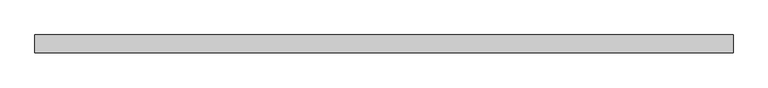
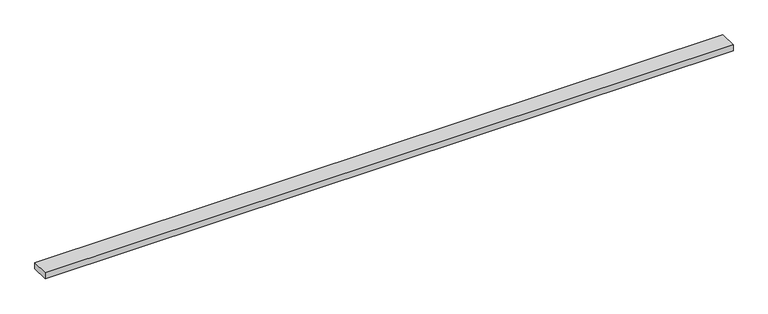
"""IFC4 building model written with IfcOpenShell, lengths in millimetres: proxy geometry, Generic Models 6:Generic Models 2:318829:Generic Models 2:318829 : Generic Models 6:Generic Models 2:318829:9 : Generic Models 6:Generic Models 2:318829:Generic Models 2:318829 : Generic Models 6:Generic Models 2:318829:300683."""

import ifcopenshell
import ifcopenshell.guid

model = None  # the IFC model being written
_history = None  # IfcOwnerHistory: only IFC2X3 demands one
_inside = {}  # id of a spatial element -> (the spatial element, [elements in it])
_under = {}  # id of a project, library or spatial element -> (it, [spatial elements below it])
_declared = {}  # id of a project -> (the project, [libraries it declares])
_typed = {}  # id of a type object -> (the type object, [elements of that type])
_made_of = {}  # id of a material, layer set ... -> (it, [elements and type objects made of it])


def new_model(schema):
    """Start an empty IFC model of exactly this schema.

    Asked for "IFC4X3", IfcOpenShell would pick the latest addendum, in which some entities
    have other attributes; the version numbers below select the first issue.
    IFC2X3 requires an IfcOwnerHistory on every rooted entity: one is made here for all.
    """
    global model, _history
    if schema == "IFC4X3":
        model = ifcopenshell.file(schema_version=(4, 3, 0, 0))
    else:
        model = ifcopenshell.file(schema=schema)
    _inside.clear()
    _under.clear()
    _declared.clear()
    _typed.clear()
    _made_of.clear()
    _history = None
    if model.schema == "IFC2X3":
        org = make("IfcOrganization", Name="unknown")
        user = make(
            "IfcPersonAndOrganization",
            ThePerson=make("IfcPerson", FamilyName="unknown"),
            TheOrganization=org,
        )
        app = make(
            "IfcApplication",
            ApplicationDeveloper=org,
            Version="unknown",
            ApplicationFullName="unknown",
            ApplicationIdentifier="unknown",
        )
        _history = make(
            "IfcOwnerHistory",
            OwningUser=user,
            OwningApplication=app,
            ChangeAction="ADDED",
            CreationDate=0,
        )
    return model


def make(cls, **values):
    """One entity of the class cls with the attributes given. An attribute that is None is left unset."""
    return model.create_entity(
        cls, **{name: value for name, value in values.items() if value is not None}
    )


def rooted(cls, **values):
    """An entity with a GlobalId (a new one), such as an element, a storey or a relation."""
    return make(cls, GlobalId=ifcopenshell.guid.new(), OwnerHistory=_history, **values)


def si_unit(unit_type, name, prefix=None):
    """IfcSIUnit, for example si_unit("LENGTHUNIT", "METRE", prefix="MILLI")."""
    return make("IfcSIUnit", UnitType=unit_type, Prefix=prefix, Name=name)


def assignment(units):
    """IfcUnitAssignment: the units of a project."""
    return None if units is None else make("IfcUnitAssignment", Units=units)


def point(xyz):
    """IfcCartesianPoint."""
    return None if xyz is None else make("IfcCartesianPoint", Coordinates=xyz)


def direction(xyz):
    """IfcDirection."""
    return None if xyz is None else make("IfcDirection", DirectionRatios=xyz)


def frame(location, z_axis=None, x_axis=None):
    """IfcAxis2Placement3D, a coordinate frame: its origin and axes. An axis left out is left unset."""
    return make(
        "IfcAxis2Placement3D",
        Location=point(location),
        Axis=direction(z_axis),
        RefDirection=direction(x_axis),
    )


def origin():
    """The frame at (0, 0, 0) with its axes left unset."""
    return frame((0.0, 0.0, 0.0))


def place(relative_to, where):
    """IfcLocalPlacement: puts the frame where relative to a parent placement (None: the world)."""
    return make(
        "IfcLocalPlacement", PlacementRelTo=relative_to, RelativePlacement=where
    )


def context(
    kind, dimensions, precision=None, world=None, true_north=None, identifier=None
):
    """IfcGeometricRepresentationContext, for example the 3D "Model" context."""
    return make(
        "IfcGeometricRepresentationContext",
        ContextIdentifier=identifier,
        ContextType=kind,
        CoordinateSpaceDimension=dimensions,
        Precision=precision,
        WorldCoordinateSystem=world,
        TrueNorth=true_north,
    )


def project(units=None, contexts=None):
    """IfcProject with its units and contexts."""
    return rooted(
        "IfcProject",
        Name="project",
        RepresentationContexts=contexts,
        UnitsInContext=assignment(units),
    )


def spatial(cls, under=None, at=None, **own):
    """A site, building, storey or space (cls), placed at a placement, below another one or the project."""
    s = rooted(cls, ObjectPlacement=at, **own)
    if under is not None:
        _under.setdefault(under.id(), (under, []))[1].append(s)
    return s


def polyline(points):
    """IfcPolyline through the points."""
    return make("IfcPolyline", Points=[point(p) for p in points])


def outline(outer, holes=None, kind="AREA"):
    """IfcArbitraryClosedProfileDef: a profile drawn as a closed curve; with holes, ...WithVoids."""
    if holes is None:
        return make("IfcArbitraryClosedProfileDef", ProfileType=kind, OuterCurve=outer)
    return make(
        "IfcArbitraryProfileDefWithVoids",
        ProfileType=kind,
        OuterCurve=outer,
        InnerCurves=holes,
    )


def extrude(swept, where, along, depth):
    """IfcExtrudedAreaSolid: the profile swept, set in the frame where, extruded along a direction by depth."""
    return make(
        "IfcExtrudedAreaSolid",
        SweptArea=swept,
        Position=where,
        ExtrudedDirection=direction(along),
        Depth=depth,
    )


def shape(context_of_items, identifier, shape_type, items):
    """IfcShapeRepresentation: the items that make up one representation, for example the "Body"."""
    return make(
        "IfcShapeRepresentation",
        ContextOfItems=context_of_items,
        RepresentationIdentifier=identifier,
        RepresentationType=shape_type,
        Items=items,
    )


def source(mapping_origin, context_of_items, identifier, shape_type, items):
    """IfcRepresentationMap: a shape defined once, which mapped items show again and again."""
    return make(
        "IfcRepresentationMap",
        MappingOrigin=mapping_origin,
        MappedRepresentation=shape(context_of_items, identifier, shape_type, items),
    )


def transform(
    local_origin,
    x_axis=None,
    y_axis=None,
    z_axis=None,
    scale=None,
    scale2=None,
    scale3=None,
    uniform=True,
):
    """IfcCartesianTransformationOperator3D, or its non-uniform kind. x_axis, y_axis, z_axis: its Axis1, 2, 3."""
    if uniform:
        return make(
            "IfcCartesianTransformationOperator3D",
            Axis1=direction(x_axis),
            Axis2=direction(y_axis),
            LocalOrigin=point(local_origin),
            Scale=scale,
            Axis3=direction(z_axis),
        )
    return make(
        "IfcCartesianTransformationOperator3DnonUniform",
        Axis1=direction(x_axis),
        Axis2=direction(y_axis),
        LocalOrigin=point(local_origin),
        Scale=scale,
        Axis3=direction(z_axis),
        Scale2=scale2,
        Scale3=scale3,
    )


def mapped(mapping_source, mapping_target):
    """IfcMappedItem: shows the shape of a source again, moved by a transform."""
    return make(
        "IfcMappedItem", MappingSource=mapping_source, MappingTarget=mapping_target
    )


def made_of(thing, what):
    """Note that an element or type object is made of a material, layer set ...; save() writes the relation."""
    if what is not None:
        _made_of.setdefault(what.id(), (what, []))[1].append(thing)
    return thing


def element(
    cls,
    number,
    at=None,
    inside=None,
    cuts=None,
    type_object=None,
    material=None,
    context=None,
    identifier="Body",
    shape_type=None,
    held_by="IfcProductDefinitionShape",
    body=None,
    shapes=None,
    **own,
):
    """One element of the class cls, such as IfcWall. Its Tag is "e" and its number.

    at: its placement. inside: the storey or other place that contains it. cuts: it is an
    opening in that element (IfcRelVoidsElement). A single representation is given by context,
    identifier, shape_type and body (its items); several are given by shapes. held_by: the class
    of the entity that holds the representations. save() writes the other relations.
    """
    e = rooted(cls, Tag="e%d" % number, ObjectPlacement=at, **own)
    if body is not None:
        shapes = [shape(context, identifier, shape_type, body)]
    if shapes is not None:
        e.Representation = make(held_by, Representations=shapes)
    if inside is not None:
        _inside.setdefault(inside.id(), (inside, []))[1].append(e)
    if cuts is not None:
        rooted(
            "IfcRelVoidsElement", RelatingBuildingElement=cuts, RelatedOpeningElement=e
        )
    if type_object is not None:
        _typed.setdefault(type_object.id(), (type_object, []))[1].append(e)
    return made_of(e, material)


def aggregate(whole, parts):
    """IfcRelAggregates: a whole, such as a stair, and the parts it consists of."""
    return rooted("IfcRelAggregates", RelatingObject=whole, RelatedObjects=parts)


def save(model, path):
    """Write the relations noted so far, then the file.

    IfcRelAggregates (storeys below a building ...), IfcRelContainedInSpatialStructure (elements
    in a storey), IfcRelDefinesByType, IfcRelAssociatesMaterial and IfcRelDeclares: one each for
    every whole, place, type object, material and project.
    """
    for whole, parts in _under.values():
        aggregate(whole, parts)
    for where, things in _inside.values():
        rooted(
            "IfcRelContainedInSpatialStructure",
            RelatedElements=things,
            RelatingStructure=where,
        )
    for kind, things in _typed.values():
        rooted("IfcRelDefinesByType", RelatedObjects=things, RelatingType=kind)
    for what, things in _made_of.values():
        rooted("IfcRelAssociatesMaterial", RelatedObjects=things, RelatingMaterial=what)
    for by, libraries in _declared.values():
        rooted("IfcRelDeclares", RelatingContext=by, RelatedDefinitions=libraries)
    model.write(path)


def generic_models_74add77e(model_context):
    return source(origin(), model_context, "Body", "SweptSolid", [
        extrude(outline(polyline([(592755.4242239, -579027.5141226), (592755.4242239, -579089.5332815), (590317.0242239, -579089.5332815), (590317.0242239, -579027.5141226), (592755.4242239, -579027.5141226)])), frame((0.0, 0.0, 4.4772173), z_axis=(0.0, 0.0, 1.0), x_axis=(1.0, 0.0, 0.0)), (0.0, 0.0, 1.0), 21.7906425),
    ])


if __name__ == "__main__":
    model = new_model("IFC4")
    model_context = context("Model", 3, world=origin())
    ifc_project = project(units=[si_unit("LENGTHUNIT", "METRE", prefix="MILLI")], contexts=[model_context])
    site = spatial("IfcSite", under=ifc_project)
    building = spatial("IfcBuilding", under=site)
    placement = place(None, origin())
    generic_models_shape = generic_models_74add77e(model_context)
    element("IfcBuildingElementProxy", 1, Name="Generic Models 6:Generic Models 2:318829:Generic Models 2:318829 : Generic Models 6:Generic Models 2:318829:9 : Generic Models 6:Generic Models 2:318829:Generic Models 2:318829 : Generic Models 6:Generic Models 2:318829:300683", ObjectType="Generic Models 6:Generic Models 2:318829:Generic Models 2:318829 : Generic Models 6:Generic Models 2:318829:9 : Generic Models 6:Generic Models 2:318829:Generic Models 2:318829 : Generic Models 6:Generic Models 2:318829:300683", at=placement, inside=building, context=model_context, shape_type="MappedRepresentation", body=[
        mapped(generic_models_shape, transform((0.0, 0.0, 0.0), x_axis=(1.0, 0.0, 0.0), y_axis=(0.0, 1.0, 0.0), z_axis=(0.0, 0.0, 1.0))),
    ])
    save(model, "model.ifc")

# Revit data of these elements
# Type "Generic Models 6:Generic Models 2:318829:Generic Models 2:318829 : Generic Models 6:Generic Models 2:318829:9 : Generic Models 6:Generic Models 2:318829:Generic Models 2:318829 : Generic Models 6:Generic Models 2:318829:300683"
#   NameOverride = "Generic Models 6:Generic Models 2:318829:Generic Models 2:318829 : Generic Models 6:Generic Models 2:318829:300683"
#   ObjectTypeOverride = "Generic Models 2:318829 : Generic Models 6:Generic Models 2:318829"
#   Reference = "Generic Models 2"
#   Tag = "300683"
# Element 1 (IfcBuildingElementProxy, "Generic Models 6:Generic Models 2:318829:Generic Models 2:318829 : Generic Models 6:Generic Models 2:318829:9 : Generic Models 6:Generic Models 2:318829:Generic Models 2:318829 : Generic Models 6:Generic Models 2:318829:300683")
#   Materials on its faces: "PRESSURE TREATED WOOD BLOCKING - SIZE AS NECESSARY"
# Materials
#   "PRESSURE TREATED WOOD BLOCKING - SIZE AS NECESSARY": class "Wood", colour RGB 144 113 62, transparency 0, Description = "Pinus Echinata", Cost = 0
